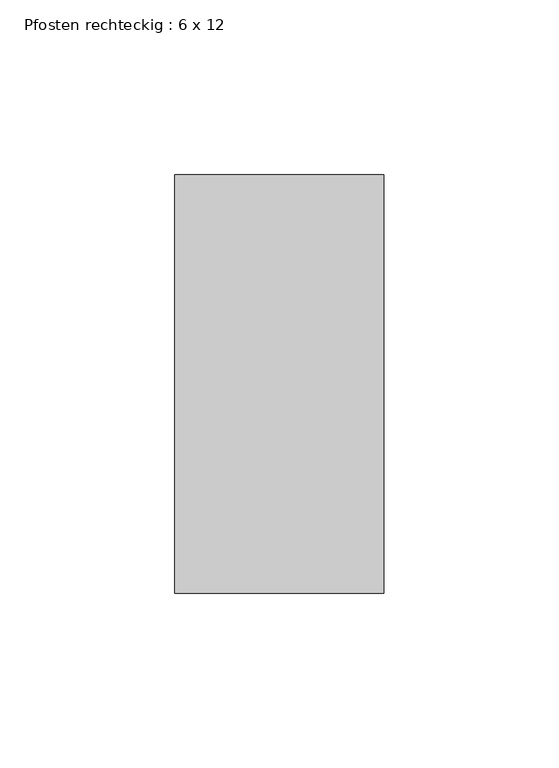
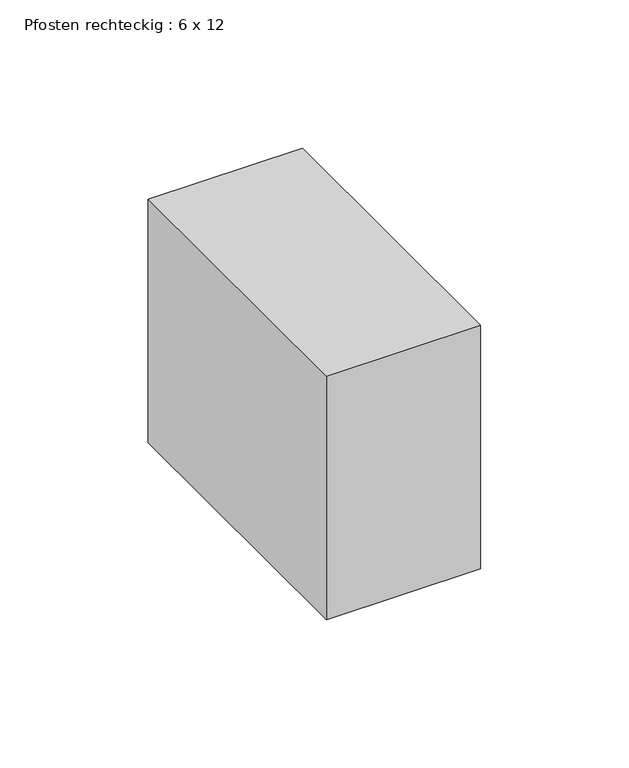
"""IFC4 building model written with IfcOpenShell, lengths in millimetres: member geometry, Pfosten rechteckig : 6 x 12."""

from ifc_helpers import new_model, si_unit, frame, origin, place, context, project, spatial, polyline, outline, extrude, source, transform, mapped, element, save


def pfosten_rechteckig_6_x_12_9d54109d(model_context):
    return source(origin(), model_context, "Body", "SweptSolid", [
        extrude(outline(polyline([(30.0, 60.0), (30.0, -60.0), (-30.0, -60.0), (-30.0, 60.0), (30.0, 60.0)])), frame((0.0, 0.0, -100.0), z_axis=(0.0, 0.0, 1.0), x_axis=(1.0, 0.0, 0.0)), (0.0, 0.0, 1.0), 100.0),
    ])


if __name__ == "__main__":
    model = new_model("IFC4")
    model_context = context("Model", 3, world=origin())
    ifc_project = project(units=[si_unit("LENGTHUNIT", "METRE", prefix="MILLI")], contexts=[model_context])
    site = spatial("IfcSite", under=ifc_project)
    building = spatial("IfcBuilding", under=site)
    placement = place(None, origin())
    pfosten_rechteckig_6_x_12_shape = pfosten_rechteckig_6_x_12_9d54109d(model_context)
    element("IfcMember", 1, ObjectType="Pfosten rechteckig : 6 x 12", at=placement, inside=building, context=model_context, shape_type="MappedRepresentation", body=[
        mapped(pfosten_rechteckig_6_x_12_shape, transform((0.0, 0.0, 0.0), x_axis=(1.0, 0.0, 0.0), y_axis=(0.0, 1.0, 0.0), z_axis=(0.0, 0.0, 1.0))),
    ])
    save(model, "model.ifc")

# Revit data of these elements
# Type "Pfosten rechteckig : 6 x 12"
#   built-in parameter 1007304 = 0.393701 (stored number, unit not read)
#   built-in parameter 1007301 = 0.0984252 (stored number, unit not read)
#   built-in parameter 1007300 = 0.0984252 (stored number, unit not read)
# Element 1 (IfcMember, "Pfosten rechteckig : 6 x 12")
#   Materials on its faces: "Metall - verzinkt"
# Materials
#   "Metall - verzinkt": class "Allgemeines", colour RGB 200 200 200, transparency 0, Cost = 0
